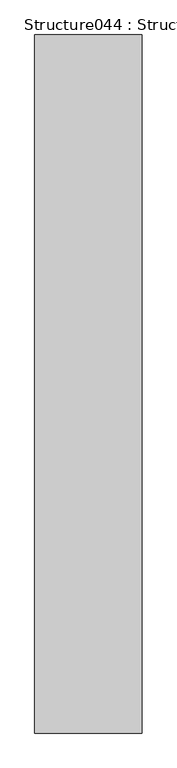
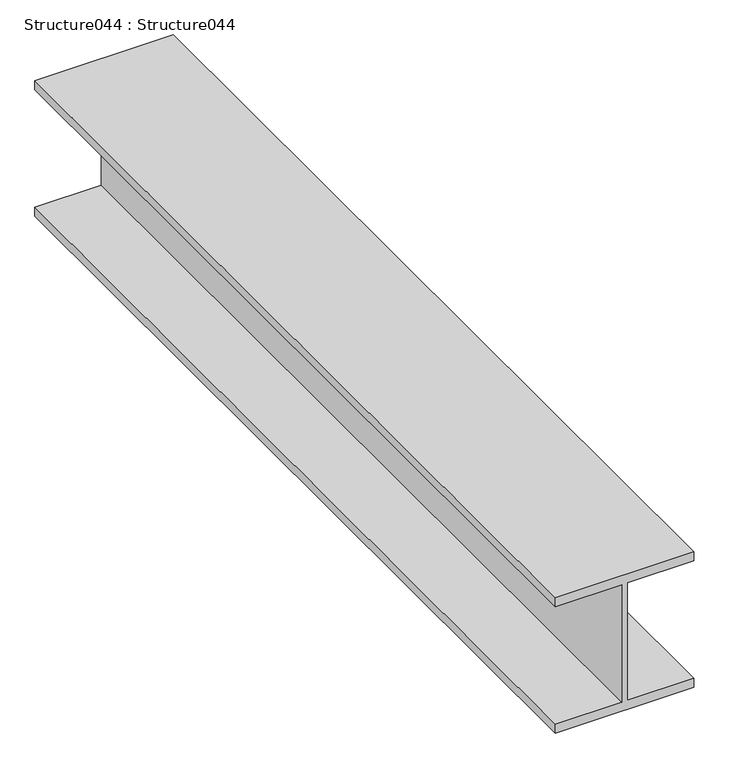
"""IFC4 building model written with IfcOpenShell, lengths in millimetres: proxy geometry, Structure044 : Structure044."""

import ifcopenshell
import ifcopenshell.guid

model = None  # the IFC model being written
_history = None  # IfcOwnerHistory: only IFC2X3 demands one
_inside = {}  # id of a spatial element -> (the spatial element, [elements in it])
_under = {}  # id of a project, library or spatial element -> (it, [spatial elements below it])
_declared = {}  # id of a project -> (the project, [libraries it declares])
_typed = {}  # id of a type object -> (the type object, [elements of that type])
_made_of = {}  # id of a material, layer set ... -> (it, [elements and type objects made of it])


def new_model(schema):
    """Start an empty IFC model of exactly this schema.

    Asked for "IFC4X3", IfcOpenShell would pick the latest addendum, in which some entities
    have other attributes; the version numbers below select the first issue.
    IFC2X3 requires an IfcOwnerHistory on every rooted entity: one is made here for all.
    """
    global model, _history
    if schema == "IFC4X3":
        model = ifcopenshell.file(schema_version=(4, 3, 0, 0))
    else:
        model = ifcopenshell.file(schema=schema)
    _inside.clear()
    _under.clear()
    _declared.clear()
    _typed.clear()
    _made_of.clear()
    _history = None
    if model.schema == "IFC2X3":
        org = make("IfcOrganization", Name="unknown")
        user = make(
            "IfcPersonAndOrganization",
            ThePerson=make("IfcPerson", FamilyName="unknown"),
            TheOrganization=org,
        )
        app = make(
            "IfcApplication",
            ApplicationDeveloper=org,
            Version="unknown",
            ApplicationFullName="unknown",
            ApplicationIdentifier="unknown",
        )
        _history = make(
            "IfcOwnerHistory",
            OwningUser=user,
            OwningApplication=app,
            ChangeAction="ADDED",
            CreationDate=0,
        )
    return model


def make(cls, **values):
    """One entity of the class cls with the attributes given. An attribute that is None is left unset."""
    return model.create_entity(
        cls, **{name: value for name, value in values.items() if value is not None}
    )


def rooted(cls, **values):
    """An entity with a GlobalId (a new one), such as an element, a storey or a relation."""
    return make(cls, GlobalId=ifcopenshell.guid.new(), OwnerHistory=_history, **values)


def si_unit(unit_type, name, prefix=None):
    """IfcSIUnit, for example si_unit("LENGTHUNIT", "METRE", prefix="MILLI")."""
    return make("IfcSIUnit", UnitType=unit_type, Prefix=prefix, Name=name)


def assignment(units):
    """IfcUnitAssignment: the units of a project."""
    return None if units is None else make("IfcUnitAssignment", Units=units)


def point(xyz):
    """IfcCartesianPoint."""
    return None if xyz is None else make("IfcCartesianPoint", Coordinates=xyz)


def direction(xyz):
    """IfcDirection."""
    return None if xyz is None else make("IfcDirection", DirectionRatios=xyz)


def frame(location, z_axis=None, x_axis=None):
    """IfcAxis2Placement3D, a coordinate frame: its origin and axes. An axis left out is left unset."""
    return make(
        "IfcAxis2Placement3D",
        Location=point(location),
        Axis=direction(z_axis),
        RefDirection=direction(x_axis),
    )


def origin():
    """The frame at (0, 0, 0) with its axes left unset."""
    return frame((0.0, 0.0, 0.0))


def place(relative_to, where):
    """IfcLocalPlacement: puts the frame where relative to a parent placement (None: the world)."""
    return make(
        "IfcLocalPlacement", PlacementRelTo=relative_to, RelativePlacement=where
    )


def context(
    kind, dimensions, precision=None, world=None, true_north=None, identifier=None
):
    """IfcGeometricRepresentationContext, for example the 3D "Model" context."""
    return make(
        "IfcGeometricRepresentationContext",
        ContextIdentifier=identifier,
        ContextType=kind,
        CoordinateSpaceDimension=dimensions,
        Precision=precision,
        WorldCoordinateSystem=world,
        TrueNorth=true_north,
    )


def project(units=None, contexts=None):
    """IfcProject with its units and contexts."""
    return rooted(
        "IfcProject",
        Name="project",
        RepresentationContexts=contexts,
        UnitsInContext=assignment(units),
    )


def spatial(cls, under=None, at=None, **own):
    """A site, building, storey or space (cls), placed at a placement, below another one or the project."""
    s = rooted(cls, ObjectPlacement=at, **own)
    if under is not None:
        _under.setdefault(under.id(), (under, []))[1].append(s)
    return s


def polyline(points):
    """IfcPolyline through the points."""
    return make("IfcPolyline", Points=[point(p) for p in points])


def outline(outer, holes=None, kind="AREA"):
    """IfcArbitraryClosedProfileDef: a profile drawn as a closed curve; with holes, ...WithVoids."""
    if holes is None:
        return make("IfcArbitraryClosedProfileDef", ProfileType=kind, OuterCurve=outer)
    return make(
        "IfcArbitraryProfileDefWithVoids",
        ProfileType=kind,
        OuterCurve=outer,
        InnerCurves=holes,
    )


def extrude(swept, where, along, depth):
    """IfcExtrudedAreaSolid: the profile swept, set in the frame where, extruded along a direction by depth."""
    return make(
        "IfcExtrudedAreaSolid",
        SweptArea=swept,
        Position=where,
        ExtrudedDirection=direction(along),
        Depth=depth,
    )


def shape(context_of_items, identifier, shape_type, items):
    """IfcShapeRepresentation: the items that make up one representation, for example the "Body"."""
    return make(
        "IfcShapeRepresentation",
        ContextOfItems=context_of_items,
        RepresentationIdentifier=identifier,
        RepresentationType=shape_type,
        Items=items,
    )


def source(mapping_origin, context_of_items, identifier, shape_type, items):
    """IfcRepresentationMap: a shape defined once, which mapped items show again and again."""
    return make(
        "IfcRepresentationMap",
        MappingOrigin=mapping_origin,
        MappedRepresentation=shape(context_of_items, identifier, shape_type, items),
    )


def transform(
    local_origin,
    x_axis=None,
    y_axis=None,
    z_axis=None,
    scale=None,
    scale2=None,
    scale3=None,
    uniform=True,
):
    """IfcCartesianTransformationOperator3D, or its non-uniform kind. x_axis, y_axis, z_axis: its Axis1, 2, 3."""
    if uniform:
        return make(
            "IfcCartesianTransformationOperator3D",
            Axis1=direction(x_axis),
            Axis2=direction(y_axis),
            LocalOrigin=point(local_origin),
            Scale=scale,
            Axis3=direction(z_axis),
        )
    return make(
        "IfcCartesianTransformationOperator3DnonUniform",
        Axis1=direction(x_axis),
        Axis2=direction(y_axis),
        LocalOrigin=point(local_origin),
        Scale=scale,
        Axis3=direction(z_axis),
        Scale2=scale2,
        Scale3=scale3,
    )


def mapped(mapping_source, mapping_target):
    """IfcMappedItem: shows the shape of a source again, moved by a transform."""
    return make(
        "IfcMappedItem", MappingSource=mapping_source, MappingTarget=mapping_target
    )


def made_of(thing, what):
    """Note that an element or type object is made of a material, layer set ...; save() writes the relation."""
    if what is not None:
        _made_of.setdefault(what.id(), (what, []))[1].append(thing)
    return thing


def element(
    cls,
    number,
    at=None,
    inside=None,
    cuts=None,
    type_object=None,
    material=None,
    context=None,
    identifier="Body",
    shape_type=None,
    held_by="IfcProductDefinitionShape",
    body=None,
    shapes=None,
    **own,
):
    """One element of the class cls, such as IfcWall. Its Tag is "e" and its number.

    at: its placement. inside: the storey or other place that contains it. cuts: it is an
    opening in that element (IfcRelVoidsElement). A single representation is given by context,
    identifier, shape_type and body (its items); several are given by shapes. held_by: the class
    of the entity that holds the representations. save() writes the other relations.
    """
    e = rooted(cls, Tag="e%d" % number, ObjectPlacement=at, **own)
    if body is not None:
        shapes = [shape(context, identifier, shape_type, body)]
    if shapes is not None:
        e.Representation = make(held_by, Representations=shapes)
    if inside is not None:
        _inside.setdefault(inside.id(), (inside, []))[1].append(e)
    if cuts is not None:
        rooted(
            "IfcRelVoidsElement", RelatingBuildingElement=cuts, RelatedOpeningElement=e
        )
    if type_object is not None:
        _typed.setdefault(type_object.id(), (type_object, []))[1].append(e)
    return made_of(e, material)


def aggregate(whole, parts):
    """IfcRelAggregates: a whole, such as a stair, and the parts it consists of."""
    return rooted("IfcRelAggregates", RelatingObject=whole, RelatedObjects=parts)


def save(model, path):
    """Write the relations noted so far, then the file.

    IfcRelAggregates (storeys below a building ...), IfcRelContainedInSpatialStructure (elements
    in a storey), IfcRelDefinesByType, IfcRelAssociatesMaterial and IfcRelDeclares: one each for
    every whole, place, type object, material and project.
    """
    for whole, parts in _under.values():
        aggregate(whole, parts)
    for where, things in _inside.values():
        rooted(
            "IfcRelContainedInSpatialStructure",
            RelatedElements=things,
            RelatingStructure=where,
        )
    for kind, things in _typed.values():
        rooted("IfcRelDefinesByType", RelatedObjects=things, RelatingType=kind)
    for what, things in _made_of.values():
        rooted("IfcRelAssociatesMaterial", RelatedObjects=things, RelatingMaterial=what)
    for by, libraries in _declared.values():
        rooted("IfcRelDeclares", RelatingContext=by, RelatedDefinitions=libraries)
    model.write(path)


def structure044_structure044_d6db8104(model_context):
    return source(origin(), model_context, "Body", "SweptSolid", [
        extrude(outline(polyline([(40092.122, -1049.2769422), (39815.77, -1049.2769422), (39815.77, -1196.4064422), (39795.196, -1196.4064422), (39795.196, -889.0664422), (39815.77, -889.0664422), (39815.77, -1036.1959422), (40092.122, -1036.1959422), (40092.122, -889.0664422), (40112.696, -889.0664422), (40112.696, -1196.4064422), (40092.122, -1196.4064422), (40092.122, -1049.2769422)])), frame((0.0, -1052.8906574, 0.0), z_axis=(0.0, 1.0, 0.0), x_axis=(0.0, 0.0, 1.0)), (0.0, 0.0, 1.0), 2000.0),
    ])


if __name__ == "__main__":
    model = new_model("IFC4")
    model_context = context("Model", 3, world=origin())
    ifc_project = project(units=[si_unit("LENGTHUNIT", "METRE", prefix="MILLI")], contexts=[model_context])
    site = spatial("IfcSite", under=ifc_project)
    building = spatial("IfcBuilding", under=site)
    placement = place(None, origin())
    structure044_structure044_shape = structure044_structure044_d6db8104(model_context)
    element("IfcBuildingElementProxy", 1, Name="Structure044 : Structure044", ObjectType="Structure044 : Structure044", at=placement, inside=building, context=model_context, shape_type="MappedRepresentation", body=[
        mapped(structure044_structure044_shape, transform((0.0, 0.0, 0.0), x_axis=(1.0, 0.0, 0.0), y_axis=(0.0, 1.0, 0.0), z_axis=(0.0, 0.0, 1.0))),
    ])
    save(model, "model.ifc")

# Revit data of these elements
# Type "Structure044 : Structure044"
#   NameOverride = "Structure044"
# Element 1 (IfcBuildingElementProxy, "Structure044 : Structure044")
#   Materials on its faces: "STEEL STRUCTURE (SEE STRUCTURAL DWGS)"
# Materials
#   "STEEL STRUCTURE (SEE STRUCTURAL DWGS)": class "Unassigned", colour RGB 128 128 128, transparency 0, Cost = 0
